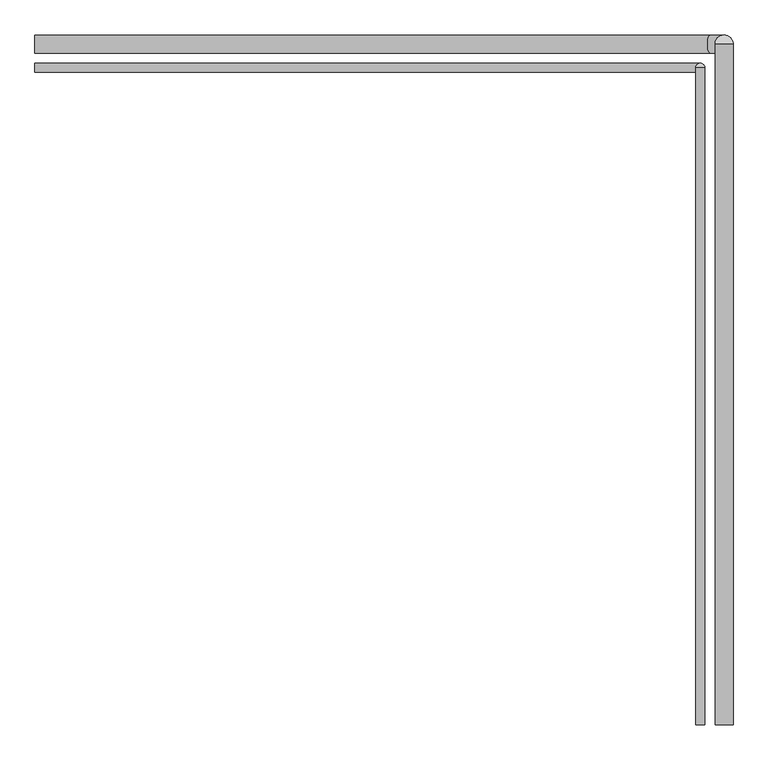
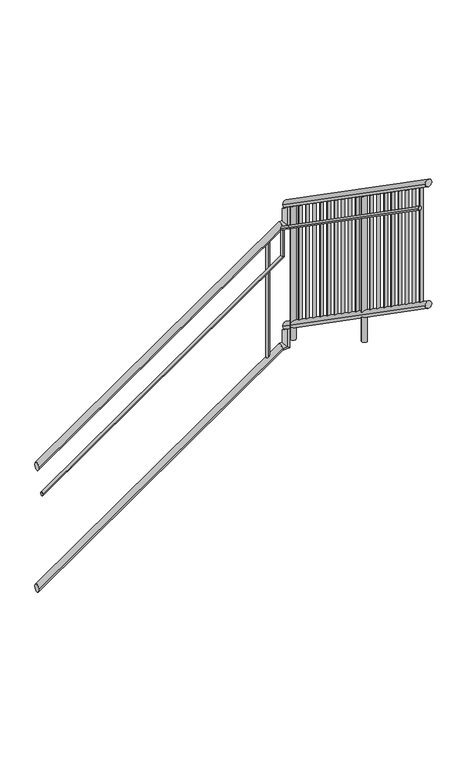
# IFC4 building model written with IfcOpenShell, lengths in millimetres: railing geometry.
# Revit data of these elements (continued)
# Materials (continued)
#   "Ferro - Pintura Esmalte": class "Pintura", colour RGB 255 255 255, transparency 0, Cost = 0
